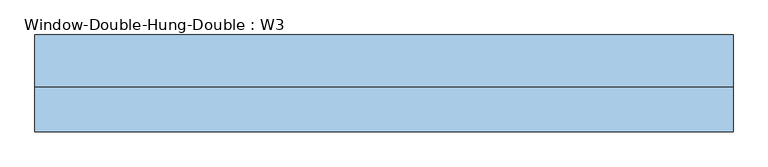
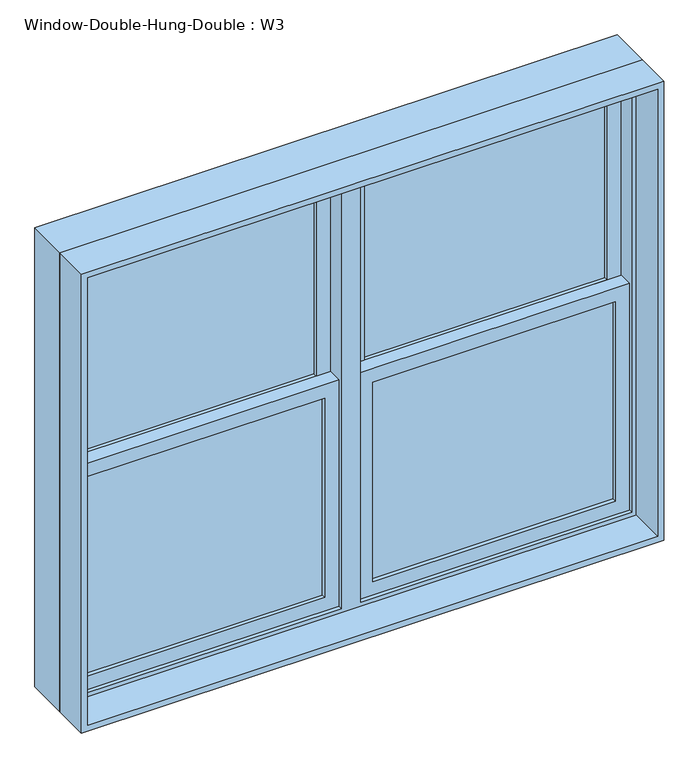
"""IFC4 building model written with IfcOpenShell, lengths in millimetres: window geometry, Window-Double-Hung-Double : W3."""

from ifc_helpers import new_model, si_unit, frame, origin, place, context, project, spatial, polyline, outline, extrude, source, transform, mapped, element, save


def window_double_hung_double_w3_63a2b5c6(model_context):
    return source(origin(), model_context, "Body", "SweptSolid", [
        extrude(outline(polyline([(2414.4, 900.0), (2414.4, -900.0), (914.4, -900.0), (914.4, 900.0), (2414.4, 900.0)]), holes=[polyline([(946.15, -868.25), (2382.65, -868.25), (2382.65, -30.1625), (946.15, -30.1625), (946.15, -868.25)]), polyline([(946.15, 868.25), (946.15, 30.1625), (2382.65, 30.1625), (2382.65, 868.25), (946.15, 868.25)])]), frame((0.0, 0.7, 0.0), z_axis=(0.0, 1.0, 0.0), x_axis=(0.0, 0.0, 1.0)), (0.0, 0.0, 1.0), 133.35),
        extrude(outline(polyline([(-823.8, 45.15), (-74.6125, 45.15), (-74.6125, 38.8), (-823.8, 38.8), (-823.8, 45.15)])), frame((0.0, 0.0, 990.6), z_axis=(0.0, 0.0, 1.0), x_axis=(1.0, 0.0, 0.0)), (0.0, 0.0, 1.0), 651.575),
        extrude(outline(polyline([(-74.6125, 32.45), (-74.6125, 26.1), (-823.8, 26.1), (-823.8, 32.45), (-74.6125, 32.45)])), frame((0.0, 0.0, 990.6), z_axis=(0.0, 0.0, 1.0), x_axis=(1.0, 0.0, 0.0)), (0.0, 0.0, 1.0), 651.575),
        extrude(outline(polyline([(-823.8, 89.6), (-74.6125, 89.6), (-74.6125, 83.25), (-823.8, 83.25), (-823.8, 89.6)])), frame((0.0, 0.0, 1686.625), z_axis=(0.0, 0.0, 1.0), x_axis=(1.0, 0.0, 0.0)), (0.0, 0.0, 1.0), 651.575),
        extrude(outline(polyline([(-74.6125, 76.9), (-74.6125, 70.55), (-823.8, 70.55), (-823.8, 76.9), (-74.6125, 76.9)])), frame((0.0, 0.0, 1686.625), z_axis=(0.0, 0.0, 1.0), x_axis=(1.0, 0.0, 0.0)), (0.0, 0.0, 1.0), 651.575),
        extrude(outline(polyline([(1686.625, -868.25), (946.15, -868.25), (946.15, -30.1625), (1686.625, -30.1625), (1686.625, -868.25)]), holes=[polyline([(1642.175, -74.6125), (990.6, -74.6125), (990.6, -823.8), (1642.175, -823.8), (1642.175, -74.6125)])]), frame((0.0, 13.4, 0.0), z_axis=(0.0, 1.0, 0.0), x_axis=(0.0, 0.0, 1.0)), (0.0, 0.0, 1.0), 44.45),
        extrude(outline(polyline([(2382.65, -868.25), (1642.175, -868.25), (1642.175, -30.1625), (2382.65, -30.1625), (2382.65, -868.25)]), holes=[polyline([(2338.2, -74.6125), (1686.625, -74.6125), (1686.625, -823.8), (2338.2, -823.8), (2338.2, -74.6125)])]), frame((0.0, 57.85, 0.0), z_axis=(0.0, 1.0, 0.0), x_axis=(0.0, 0.0, 1.0)), (0.0, 0.0, 1.0), 44.45),
        extrude(outline(polyline([(823.8, 45.15), (823.8, 38.8), (74.6125, 38.8), (74.6125, 45.15), (823.8, 45.15)])), frame((0.0, 0.0, 990.6), z_axis=(0.0, 0.0, 1.0), x_axis=(1.0, 0.0, 0.0)), (0.0, 0.0, 1.0), 651.575),
        extrude(outline(polyline([(74.6125, 32.45), (823.8, 32.45), (823.8, 26.1), (74.6125, 26.1), (74.6125, 32.45)])), frame((0.0, 0.0, 990.6), z_axis=(0.0, 0.0, 1.0), x_axis=(1.0, 0.0, 0.0)), (0.0, 0.0, 1.0), 651.575),
        extrude(outline(polyline([(823.8, 89.6), (823.8, 83.25), (74.6125, 83.25), (74.6125, 89.6), (823.8, 89.6)])), frame((0.0, 0.0, 1686.625), z_axis=(0.0, 0.0, 1.0), x_axis=(1.0, 0.0, 0.0)), (0.0, 0.0, 1.0), 651.575),
        extrude(outline(polyline([(74.6125, 76.9), (823.8, 76.9), (823.8, 70.55), (74.6125, 70.55), (74.6125, 76.9)])), frame((0.0, 0.0, 1686.625), z_axis=(0.0, 0.0, 1.0), x_axis=(1.0, 0.0, 0.0)), (0.0, 0.0, 1.0), 651.575),
        extrude(outline(polyline([(1686.625, 30.1625), (946.15, 30.1625), (946.15, 868.25), (1686.625, 868.25), (1686.625, 30.1625)]), holes=[polyline([(1642.175, 823.8), (990.6, 823.8), (990.6, 74.6125), (1642.175, 74.6125), (1642.175, 823.8)])]), frame((0.0, 13.4, 0.0), z_axis=(0.0, 1.0, 0.0), x_axis=(0.0, 0.0, 1.0)), (0.0, 0.0, 1.0), 44.45),
        extrude(outline(polyline([(2382.65, 30.1625), (1642.175, 30.1625), (1642.175, 868.25), (2382.65, 868.25), (2382.65, 30.1625)]), holes=[polyline([(2338.2, 823.8), (1686.625, 823.8), (1686.625, 74.6125), (2338.2, 74.6125), (2338.2, 823.8)])]), frame((0.0, 57.85, 0.0), z_axis=(0.0, 1.0, 0.0), x_axis=(0.0, 0.0, 1.0)), (0.0, 0.0, 1.0), 44.45),
        extrude(outline(polyline([(2414.4, 900.0), (2414.4, -900.0), (914.4, -900.0), (914.4, 900.0), (2414.4, 900.0)]), holes=[polyline([(2395.35, 880.95), (933.45, 880.95), (933.45, -880.95), (2395.35, -880.95), (2395.35, 880.95)])]), frame((0.0, -115.0, 0.0), z_axis=(0.0, 1.0, 0.0), x_axis=(0.0, 0.0, 1.0)), (0.0, 0.0, 1.0), 115.7),
    ])


if __name__ == "__main__":
    model = new_model("IFC4")
    model_context = context("Model", 3, world=origin())
    ifc_project = project(units=[si_unit("LENGTHUNIT", "METRE", prefix="MILLI")], contexts=[model_context])
    site = spatial("IfcSite", under=ifc_project)
    building = spatial("IfcBuilding", under=site)
    placement = place(None, origin())
    window_double_hung_double_w3_shape = window_double_hung_double_w3_63a2b5c6(model_context)
    element("IfcWindow", 1, ObjectType="Window-Double-Hung-Double : W3", at=placement, inside=building, context=model_context, shape_type="MappedRepresentation", body=[
        mapped(window_double_hung_double_w3_shape, transform((0.0, 0.0, 0.0), x_axis=(1.0, 0.0, 0.0), y_axis=(0.0, 1.0, 0.0), z_axis=(0.0, 0.0, 1.0))),
    ])
    save(model, "model.ifc")

# Revit data of these elements
# Type "Window-Double-Hung-Double : W3"
#   Type Mark = "33"
#   Fire Rating = "0.5h"
#   Construction Type Id = "DG-DR"
#   Assembly Code = "B2020100"
#   Analytic Construction = "Double glazing - domestic"
#   Wall Thickness [instance default] = 15.24 cm
#   Window Inset [instance default] = 0 cm
#   Visual Light Transmittance = 0.81
#   Thermal Resistance (R) = 0.319569 (m²·K)/W
#   Solar Heat Gain Coefficient = 0.76
#   Muntin Width = 74.9188 cm
#   Muntin Height = 65.1575 cm
#   Interior Wall Closure [instance default] = 3.81 cm
#   Rough Width = 181.27 cm
#   Rough Height = 151.27 cm
#   Frame Extension [instance default] = 3.175 cm
#   Exterior Wall Closure [instance default] = 1.27 cm
#   Extension Jamb [instance default] = 3.81 cm
#   Heat Transfer Coefficient (U) = 3.12929 W/(m²·K)
#   Height = 150 cm
#   Width = 180 cm
#   Top Muntin Visibility = yes
#   Indicator Visibility [instance default] = yes
#   Extension Jamb Visibility [instance default] = yes
#   Interior Trim Visibility [instance default] = yes
#   Exterior Trim Visibility [instance default] = yes
#   Bottom Muntin Visibility = yes
#   Muntin Pattern = Muntin Pattern_2x2 : Muntin Pattern_2x2
#   Interior Trim Material = Wood - Stained
#   Interior Trim = Trim-Window-Interior-Flat : Picture Frame
#   Exterior Trim Material = Clad - White
#   Exterior Trim = Trim-Window-Exterior-Flat : with Sill
#   Glass Panel Material = Glass
#   Exterior Frame Material = Clad - White
#   Interior Frame Material = Wood - Stained
#   Wall Closure = (empty or 0)
# Element 1 (IfcWindow, "Window-Double-Hung-Double : W3")
#   Wall Thickness = 23 cm
#   Extension Jamb = 11.57 cm
#   Materials on its faces: "Wood - Stained", "Glass", "Clad - White"
# Materials
#   "Wood - Stained": class "Wood", colour RGB 224 178 126, transparency 0, Cost = 0
#   "Clad - White": class "Wood", colour RGB 242 242 238, transparency 0, Cost = 0
#   "Glass": class "Glass", colour RGB 0 128 192, transparency 0.9, Description = "Soda Lime Glass", Cost = 0
